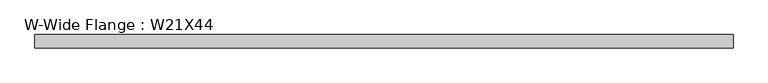
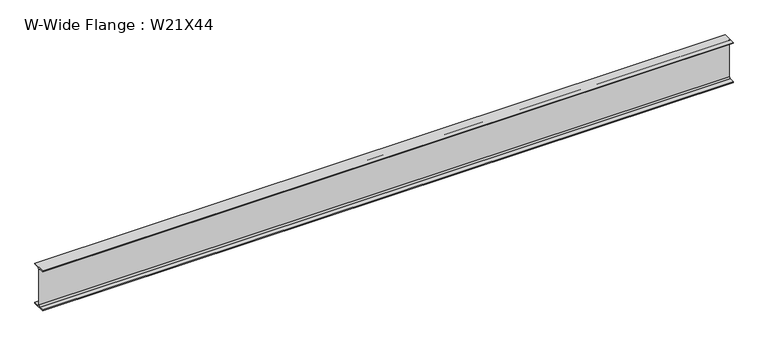
"""IFC4 building model written with IfcOpenShell, lengths in millimetres: beam geometry, W-Wide Flange : W21X44."""

from ifc_helpers import new_model, si_unit, point, frame, frame_2d, origin, place, context, project, spatial, polyline, circle_curve, trimmed, segment, composite_curve, outline, extrude, source, transform, mapped, element, save


def w_wide_flange_w21x44_bd9b7f00(model_context):
    return source(origin(), model_context, "Body", "SweptSolid", [
        extrude(outline(composite_curve([segment(polyline([(82.55, -251.46), (82.55, -262.89), (-82.55, -262.89), (-82.55, -251.46), (-21.59, -251.46)]), True, "CONTINUOUS"), segment(trimmed(circle_curve(frame_2d((-21.59, -234.315)), 17.145), [point((-21.59, -251.46))], [point((-4.445, -234.315))], True, "CARTESIAN"), True, "CONTINUOUS"), segment(polyline([(-4.445, -234.315), (-4.445, 234.315)]), True, "CONTINUOUS"), segment(trimmed(circle_curve(frame_2d((-21.59, 234.315)), 17.145), [point((-4.445, 234.315))], [point((-21.59, 251.46))], True, "CARTESIAN"), True, "CONTINUOUS"), segment(polyline([(-21.59, 251.46), (-82.55, 251.46), (-82.55, 262.89), (82.55, 262.89), (82.55, 251.46), (21.59, 251.46)]), True, "CONTINUOUS"), segment(trimmed(circle_curve(frame_2d((21.59, 234.315)), 17.145), [point((21.59, 251.46))], [point((4.445, 234.315))], True, "CARTESIAN"), True, "CONTINUOUS"), segment(polyline([(4.445, 234.315), (4.445, -234.315)]), True, "CONTINUOUS"), segment(trimmed(circle_curve(frame_2d((21.59, -234.315)), 17.145), [point((4.445, -234.315))], [point((21.59, -251.46))], True, "CARTESIAN"), True, "CONTINUOUS"), segment(polyline([(21.59, -251.46), (82.55, -251.46)]), True, "CONTINUOUS")], self_intersect=False)), frame((-4221.1128906, 0.0, 0.0), z_axis=(1.0, 0.0, 0.0), x_axis=(0.0, 1.0, 0.0)), (0.0, 0.0, 1.0), 8577.1632812),
    ])


if __name__ == "__main__":
    model = new_model("IFC4")
    model_context = context("Model", 3, world=origin())
    ifc_project = project(units=[si_unit("LENGTHUNIT", "METRE", prefix="MILLI")], contexts=[model_context])
    site = spatial("IfcSite", under=ifc_project)
    building = spatial("IfcBuilding", under=site)
    placement = place(None, origin())
    w_wide_flange_w21x44_shape = w_wide_flange_w21x44_bd9b7f00(model_context)
    element("IfcBeam", 1, ObjectType="W-Wide Flange : W21X44", at=placement, inside=building, context=model_context, shape_type="MappedRepresentation", body=[
        mapped(w_wide_flange_w21x44_shape, transform((0.0, 0.0, 0.0), x_axis=(1.0, 0.0, 0.0), y_axis=(0.0, 1.0, 0.0), z_axis=(0.0, 0.0, 1.0))),
    ])
    save(model, "model.ifc")

# Revit data of these elements
# Type "W-Wide Flange : W21X44"
#   Assembly Code = "B10"
#   W = 44
#   Length [instance default] = 1524 mm
#   bf = 165.1 mm
#   d = 525.78 mm
#   k = 28.575 mm
#   k2 = 17.145 mm
#   tf = 11.43 mm
#   tw = 8.89 mm
#   A = 0.00838708 m²
#   Structural Material [instance default] = Steel ASTM A992
# Element 1 (IfcBeam, "W-Wide Flange : W21X44")
#   Structural Material = Aluminum, Anodized Red
#   Materials on its faces: "Aluminum, Anodized Red"
# Materials
#   "Steel ASTM A992": class "Metal", colour RGB 128 0 0, transparency 0, Description = "Structural steel 50ksi", Cost = 0
#   "Aluminum, Anodized Red": class "Metal", colour RGB 120 120 120, transparency 0, Description = "Anodized aluminum, red", Cost = 0
